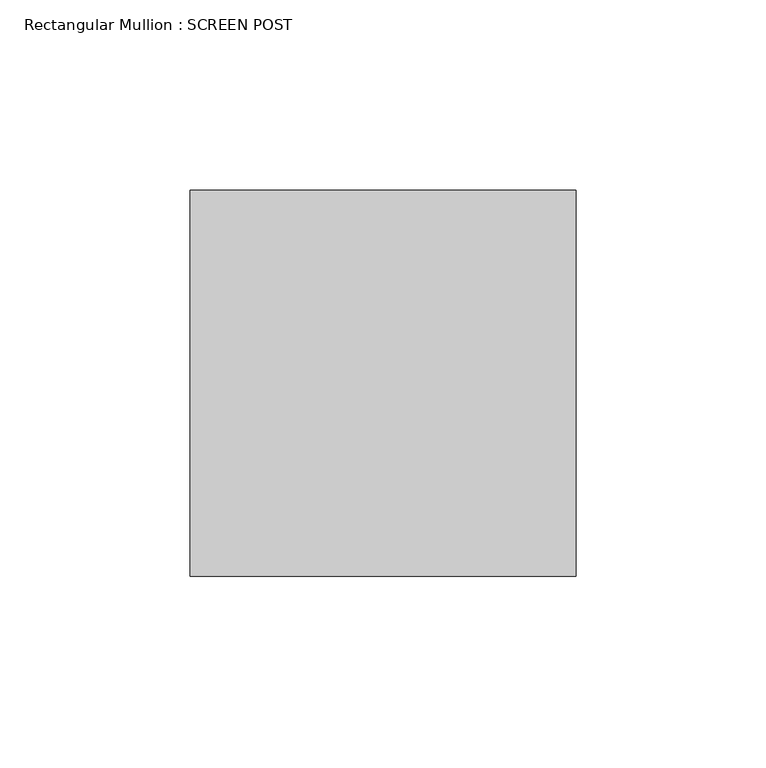
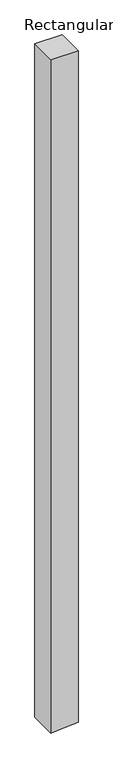
"""IFC4 building model written with IfcOpenShell, lengths in millimetres: member geometry, Rectangular Mullion : SCREEN POST."""

import ifcopenshell
import ifcopenshell.guid

model = None  # the IFC model being written
_history = None  # IfcOwnerHistory: only IFC2X3 demands one
_inside = {}  # id of a spatial element -> (the spatial element, [elements in it])
_under = {}  # id of a project, library or spatial element -> (it, [spatial elements below it])
_declared = {}  # id of a project -> (the project, [libraries it declares])
_typed = {}  # id of a type object -> (the type object, [elements of that type])
_made_of = {}  # id of a material, layer set ... -> (it, [elements and type objects made of it])


def new_model(schema):
    """Start an empty IFC model of exactly this schema.

    Asked for "IFC4X3", IfcOpenShell would pick the latest addendum, in which some entities
    have other attributes; the version numbers below select the first issue.
    IFC2X3 requires an IfcOwnerHistory on every rooted entity: one is made here for all.
    """
    global model, _history
    if schema == "IFC4X3":
        model = ifcopenshell.file(schema_version=(4, 3, 0, 0))
    else:
        model = ifcopenshell.file(schema=schema)
    _inside.clear()
    _under.clear()
    _declared.clear()
    _typed.clear()
    _made_of.clear()
    _history = None
    if model.schema == "IFC2X3":
        org = make("IfcOrganization", Name="unknown")
        user = make(
            "IfcPersonAndOrganization",
            ThePerson=make("IfcPerson", FamilyName="unknown"),
            TheOrganization=org,
        )
        app = make(
            "IfcApplication",
            ApplicationDeveloper=org,
            Version="unknown",
            ApplicationFullName="unknown",
            ApplicationIdentifier="unknown",
        )
        _history = make(
            "IfcOwnerHistory",
            OwningUser=user,
            OwningApplication=app,
            ChangeAction="ADDED",
            CreationDate=0,
        )
    return model


def make(cls, **values):
    """One entity of the class cls with the attributes given. An attribute that is None is left unset."""
    return model.create_entity(
        cls, **{name: value for name, value in values.items() if value is not None}
    )


def rooted(cls, **values):
    """An entity with a GlobalId (a new one), such as an element, a storey or a relation."""
    return make(cls, GlobalId=ifcopenshell.guid.new(), OwnerHistory=_history, **values)


def si_unit(unit_type, name, prefix=None):
    """IfcSIUnit, for example si_unit("LENGTHUNIT", "METRE", prefix="MILLI")."""
    return make("IfcSIUnit", UnitType=unit_type, Prefix=prefix, Name=name)


def assignment(units):
    """IfcUnitAssignment: the units of a project."""
    return None if units is None else make("IfcUnitAssignment", Units=units)


def point(xyz):
    """IfcCartesianPoint."""
    return None if xyz is None else make("IfcCartesianPoint", Coordinates=xyz)


def direction(xyz):
    """IfcDirection."""
    return None if xyz is None else make("IfcDirection", DirectionRatios=xyz)


def frame(location, z_axis=None, x_axis=None):
    """IfcAxis2Placement3D, a coordinate frame: its origin and axes. An axis left out is left unset."""
    return make(
        "IfcAxis2Placement3D",
        Location=point(location),
        Axis=direction(z_axis),
        RefDirection=direction(x_axis),
    )


def origin():
    """The frame at (0, 0, 0) with its axes left unset."""
    return frame((0.0, 0.0, 0.0))


def place(relative_to, where):
    """IfcLocalPlacement: puts the frame where relative to a parent placement (None: the world)."""
    return make(
        "IfcLocalPlacement", PlacementRelTo=relative_to, RelativePlacement=where
    )


def context(
    kind, dimensions, precision=None, world=None, true_north=None, identifier=None
):
    """IfcGeometricRepresentationContext, for example the 3D "Model" context."""
    return make(
        "IfcGeometricRepresentationContext",
        ContextIdentifier=identifier,
        ContextType=kind,
        CoordinateSpaceDimension=dimensions,
        Precision=precision,
        WorldCoordinateSystem=world,
        TrueNorth=true_north,
    )


def project(units=None, contexts=None):
    """IfcProject with its units and contexts."""
    return rooted(
        "IfcProject",
        Name="project",
        RepresentationContexts=contexts,
        UnitsInContext=assignment(units),
    )


def spatial(cls, under=None, at=None, **own):
    """A site, building, storey or space (cls), placed at a placement, below another one or the project."""
    s = rooted(cls, ObjectPlacement=at, **own)
    if under is not None:
        _under.setdefault(under.id(), (under, []))[1].append(s)
    return s


def polyline(points):
    """IfcPolyline through the points."""
    return make("IfcPolyline", Points=[point(p) for p in points])


def outline(outer, holes=None, kind="AREA"):
    """IfcArbitraryClosedProfileDef: a profile drawn as a closed curve; with holes, ...WithVoids."""
    if holes is None:
        return make("IfcArbitraryClosedProfileDef", ProfileType=kind, OuterCurve=outer)
    return make(
        "IfcArbitraryProfileDefWithVoids",
        ProfileType=kind,
        OuterCurve=outer,
        InnerCurves=holes,
    )


def extrude(swept, where, along, depth):
    """IfcExtrudedAreaSolid: the profile swept, set in the frame where, extruded along a direction by depth."""
    return make(
        "IfcExtrudedAreaSolid",
        SweptArea=swept,
        Position=where,
        ExtrudedDirection=direction(along),
        Depth=depth,
    )


def shape(context_of_items, identifier, shape_type, items):
    """IfcShapeRepresentation: the items that make up one representation, for example the "Body"."""
    return make(
        "IfcShapeRepresentation",
        ContextOfItems=context_of_items,
        RepresentationIdentifier=identifier,
        RepresentationType=shape_type,
        Items=items,
    )


def source(mapping_origin, context_of_items, identifier, shape_type, items):
    """IfcRepresentationMap: a shape defined once, which mapped items show again and again."""
    return make(
        "IfcRepresentationMap",
        MappingOrigin=mapping_origin,
        MappedRepresentation=shape(context_of_items, identifier, shape_type, items),
    )


def transform(
    local_origin,
    x_axis=None,
    y_axis=None,
    z_axis=None,
    scale=None,
    scale2=None,
    scale3=None,
    uniform=True,
):
    """IfcCartesianTransformationOperator3D, or its non-uniform kind. x_axis, y_axis, z_axis: its Axis1, 2, 3."""
    if uniform:
        return make(
            "IfcCartesianTransformationOperator3D",
            Axis1=direction(x_axis),
            Axis2=direction(y_axis),
            LocalOrigin=point(local_origin),
            Scale=scale,
            Axis3=direction(z_axis),
        )
    return make(
        "IfcCartesianTransformationOperator3DnonUniform",
        Axis1=direction(x_axis),
        Axis2=direction(y_axis),
        LocalOrigin=point(local_origin),
        Scale=scale,
        Axis3=direction(z_axis),
        Scale2=scale2,
        Scale3=scale3,
    )


def mapped(mapping_source, mapping_target):
    """IfcMappedItem: shows the shape of a source again, moved by a transform."""
    return make(
        "IfcMappedItem", MappingSource=mapping_source, MappingTarget=mapping_target
    )


def made_of(thing, what):
    """Note that an element or type object is made of a material, layer set ...; save() writes the relation."""
    if what is not None:
        _made_of.setdefault(what.id(), (what, []))[1].append(thing)
    return thing


def element(
    cls,
    number,
    at=None,
    inside=None,
    cuts=None,
    type_object=None,
    material=None,
    context=None,
    identifier="Body",
    shape_type=None,
    held_by="IfcProductDefinitionShape",
    body=None,
    shapes=None,
    **own,
):
    """One element of the class cls, such as IfcWall. Its Tag is "e" and its number.

    at: its placement. inside: the storey or other place that contains it. cuts: it is an
    opening in that element (IfcRelVoidsElement). A single representation is given by context,
    identifier, shape_type and body (its items); several are given by shapes. held_by: the class
    of the entity that holds the representations. save() writes the other relations.
    """
    e = rooted(cls, Tag="e%d" % number, ObjectPlacement=at, **own)
    if body is not None:
        shapes = [shape(context, identifier, shape_type, body)]
    if shapes is not None:
        e.Representation = make(held_by, Representations=shapes)
    if inside is not None:
        _inside.setdefault(inside.id(), (inside, []))[1].append(e)
    if cuts is not None:
        rooted(
            "IfcRelVoidsElement", RelatingBuildingElement=cuts, RelatedOpeningElement=e
        )
    if type_object is not None:
        _typed.setdefault(type_object.id(), (type_object, []))[1].append(e)
    return made_of(e, material)


def aggregate(whole, parts):
    """IfcRelAggregates: a whole, such as a stair, and the parts it consists of."""
    return rooted("IfcRelAggregates", RelatingObject=whole, RelatedObjects=parts)


def save(model, path):
    """Write the relations noted so far, then the file.

    IfcRelAggregates (storeys below a building ...), IfcRelContainedInSpatialStructure (elements
    in a storey), IfcRelDefinesByType, IfcRelAssociatesMaterial and IfcRelDeclares: one each for
    every whole, place, type object, material and project.
    """
    for whole, parts in _under.values():
        aggregate(whole, parts)
    for where, things in _inside.values():
        rooted(
            "IfcRelContainedInSpatialStructure",
            RelatedElements=things,
            RelatingStructure=where,
        )
    for kind, things in _typed.values():
        rooted("IfcRelDefinesByType", RelatedObjects=things, RelatingType=kind)
    for what, things in _made_of.values():
        rooted("IfcRelAssociatesMaterial", RelatedObjects=things, RelatingMaterial=what)
    for by, libraries in _declared.values():
        rooted("IfcRelDeclares", RelatingContext=by, RelatedDefinitions=libraries)
    model.write(path)


def rectangular_mullion_screen_post_438fc00e(model_context):
    return source(origin(), model_context, "Body", "SweptSolid", [
        extrude(outline(polyline([(0.0, 50.8), (0.0, -50.8), (-2647.591053, -50.8), (-2644.8078487, -6.3490391), (-2641.2295808, 50.8), (0.0, 50.8)])), frame((0.0, -50.8, 0.0), z_axis=(0.0, 1.0, 0.0), x_axis=(0.0, 0.0, 1.0)), (0.0, 0.0, 1.0), 101.6),
    ])


if __name__ == "__main__":
    model = new_model("IFC4")
    model_context = context("Model", 3, world=origin())
    ifc_project = project(units=[si_unit("LENGTHUNIT", "METRE", prefix="MILLI")], contexts=[model_context])
    site = spatial("IfcSite", under=ifc_project)
    building = spatial("IfcBuilding", under=site)
    placement = place(None, origin())
    rectangular_mullion_screen_post_shape = rectangular_mullion_screen_post_438fc00e(model_context)
    element("IfcMember", 1, ObjectType="Rectangular Mullion : SCREEN POST", at=placement, inside=building, context=model_context, shape_type="MappedRepresentation", body=[
        mapped(rectangular_mullion_screen_post_shape, transform((0.0, 0.0, 0.0), x_axis=(1.0, 0.0, 0.0), y_axis=(0.0, 1.0, 0.0), z_axis=(0.0, 0.0, 1.0))),
    ])
    save(model, "model.ifc")

# Revit data of these elements
# Type "Rectangular Mullion : SCREEN POST"
#   built-in parameter 1007304 = 0.333333 (stored number, unit not read)
#   built-in parameter 1007301 = 0.166667 (stored number, unit not read)
#   built-in parameter 1007300 = 0.166667 (stored number, unit not read)
# Element 1 (IfcMember, "Rectangular Mullion : SCREEN POST")
#   Materials on its faces: "SCREEN PORCH FRAMING"
# Materials
#   "SCREEN PORCH FRAMING": class "Wood", colour RGB 164 134 123, transparency 0, Description = "Pinus Echinata", Cost = 0
